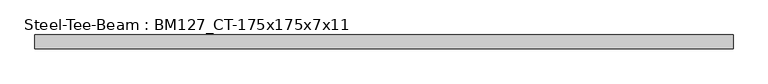
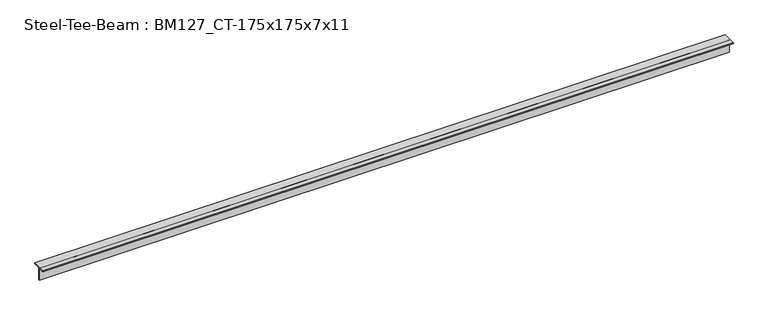
"""IFC4 building model written with IfcOpenShell, lengths in millimetres: beam geometry, Steel-Tee-Beam : BM127_CT-175x175x7x11."""

from ifc_helpers import new_model, si_unit, point, frame, frame_2d, origin, place, context, project, spatial, polyline, circle_curve, trimmed, segment, composite_curve, outline, extrude, source, transform, mapped, element, save


def steel_tee_beam_bm127_ct_175x175x7x11_7511bb12(model_context):
    return source(origin(), model_context, "Body", "SweptSolid", [
        extrude(outline(composite_curve([segment(polyline([(87.5, 87.5), (87.5, 76.5), (17.5, 76.5)]), True, "CONTINUOUS"), segment(trimmed(circle_curve(frame_2d((17.5, 62.5)), 14.0), [point((17.5, 76.5))], [point((3.5, 62.5))], True, "CARTESIAN"), True, "CONTINUOUS"), segment(polyline([(3.5, 62.5), (3.5, -87.5), (-3.5, -87.5), (-3.5, 62.5)]), True, "CONTINUOUS"), segment(trimmed(circle_curve(frame_2d((-17.5, 62.5)), 14.0), [point((-3.5, 62.5))], [point((-17.5, 76.5))], True, "CARTESIAN"), True, "CONTINUOUS"), segment(polyline([(-17.5, 76.5), (-87.5, 76.5), (-87.5, 87.5), (87.5, 87.5)]), True, "CONTINUOUS")], self_intersect=False)), frame((-4427.0238227, 0.0, 0.0), z_axis=(1.0, 0.0, 0.0), x_axis=(0.0, 1.0, 0.0)), (0.0, 0.0, 1.0), 8723.5825238),
    ])


if __name__ == "__main__":
    model = new_model("IFC4")
    model_context = context("Model", 3, world=origin())
    ifc_project = project(units=[si_unit("LENGTHUNIT", "METRE", prefix="MILLI")], contexts=[model_context])
    site = spatial("IfcSite", under=ifc_project)
    building = spatial("IfcBuilding", under=site)
    placement = place(None, origin())
    steel_tee_beam_bm127_ct_175x175x7x11_shape = steel_tee_beam_bm127_ct_175x175x7x11_7511bb12(model_context)
    element("IfcBeam", 1, ObjectType="Steel-Tee-Beam : BM127_CT-175x175x7x11", at=placement, inside=building, context=model_context, shape_type="MappedRepresentation", body=[
        mapped(steel_tee_beam_bm127_ct_175x175x7x11_shape, transform((0.0, 0.0, 0.0), x_axis=(1.0, 0.0, 0.0), y_axis=(0.0, 1.0, 0.0), z_axis=(0.0, 0.0, 1.0))),
    ])
    save(model, "model.ifc")

# Revit data of these elements
# Type "Steel-Tee-Beam : BM127_CT-175x175x7x11"
#   Surface Area = 0.00 m²/m
#   Section Area = 31.57 cm²
#   Mass per Unit Length = 24.80 kg/m
#   Length [instance default] = 1524 mm
#   bf = 175 mm
#   d = 175 mm
#   k = 25 mm
#   kr = 14 mm
#   tf = 11 mm
#   tw = 7 mm
#   hec_material4 [instance default] = none
#   hec_material3 [instance default] = none
#   hec_material2 [instance default] = none
#   hec_material1 [instance default] = none
#   Structural Material [instance default] = Steel, 45-345
#   Assembly Code = ""
# Element 1 (IfcBeam, "Steel-Tee-Beam : BM127_CT-175x175x7x11")
#   hec_material3 = F01AC000-00002_Building/Shelter Fire Proofing Work_Intumescent Coating Type_1 hr. rating (UL 1709))
#   hec_material2 = S01AA010-00002_Main Steel Structure Fabrication Work_Shelter/Building_Steel Painting/Coating_for Fireproofed Steel Surface, Surface Preparation & Primer Coat
#   hec_material1 = S03AA029-00001_Main Steel Structure Erection Work_Shelter/Building_Light Steel
#   Structural Material = S01AA003-00001_Main Steel Structure Fabrication Work_Shelter/Building_Light Steel - Standard
#   Materials on its faces: "S01AA003-00001_Main Steel Structure Fabrication Work_Shelter/Building_Light Steel - Standard"
# Materials
#   "Steel, 45-345": class "Metal", colour RGB 189 187 185, transparency 0, Description = "Steel 345 MPa", Cost = 0
#   "S01AA003-00001_Main Steel Structure Fabrication Work_Shelter/Building_Light Steel - Standard": class "Metal", colour RGB 120 120 120, transparency 0, Comments = "(30KG/M>Weight)", Description = "Structural steel 50ksi", W00) Work Master Code = "S01AA003-00001", W01) Work Master_Lv1 = "Main Steel Structure Fabrication Work", W02) Work Master_Lv2 = "Shelter/Building", W03) Work Master_Spec.1 = "Light Steel - Standard (30KG/M>Weight)", Cost = 0
#   "F01AC000-00002_Building/Shelter Fire Proofing Work_Intumescent Coating Type_1 hr. rating (UL 1709))": class "Metal", colour RGB 255 128 128, transparency 0, Description = "Paint finished steel", W00) Work Master Code = "F01AC000-00002", W01) Work Master_Lv1 = "Building/Shelter Fire Proofing Work", W02) Work Master_Lv2 = "Intumescent Coating Type", W03) Work Master_Spec.1 = "1 hr. rating (UL 1709)", Cost = 0
#   "S01AA010-00002_Main Steel Structure Fabrication Work_Shelter/Building_Steel Painting/Coating_for Fireproofed Steel Surface, Surface Preparation & Primer Coat": class "Metal", colour RGB 120 120 120, transparency 0, Description = "Paint finished steel", W00) Work Master Code = "SS01AA010-00002", W01) Work Master_Lv1 = "Main Steel Structure Fabrication Work", W02) Work Master_Lv2 = "Shelter/Building", W03) Work Master_Spec.1 = "Steel Painting/Coating", W04) Work Master_Spec.2 = "for Fireproofed Steel Surface, Surface Preparation & Primer Coat", Cost = 0
#   "S03AA029-00001_Main Steel Structure Erection Work_Shelter/Building_Light Steel": class "Metal", colour RGB 120 120 120, transparency 0, Comments = "(30KG/M>Weight)", Description = "Structural steel 50ksi", W00) Work Master Code = "S03AA029-00001", W01) Work Master_Lv1 = "Main Steel Structure Erection Work", W02) Work Master_Lv2 = "Shelter/Building", W03) Work Master_Spec.1 = "Light Steel (30KG/M>Weight)", Cost = 0
